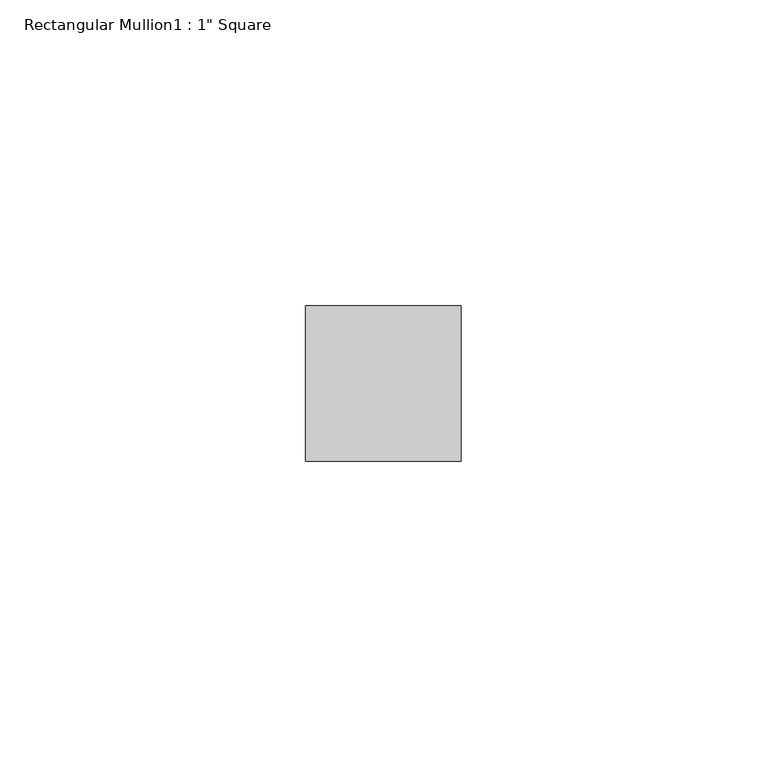
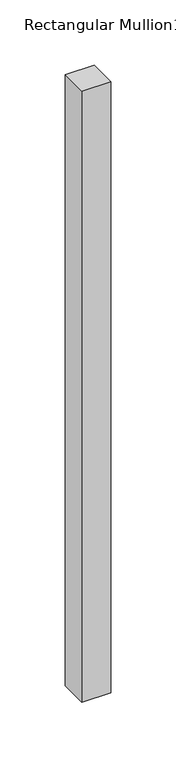
"""IFC4 building model written with IfcOpenShell, lengths in millimetres: member geometry."""

from ifc_helpers import new_model, si_unit, frame, origin, place, context, project, spatial, polyline, outline, extrude, source, transform, mapped, element, save


def member_8ca96f9c(model_context):
    return source(origin(), model_context, "Body", "SweptSolid", [
        extrude(outline(polyline([(12.7, -19.05), (12.7, -44.45), (-12.7, -44.45), (-12.7, -19.05), (12.7, -19.05)])), frame((0.0, 0.0, -571.5), z_axis=(0.0, 0.0, 1.0), x_axis=(1.0, 0.0, 0.0)), (0.0, 0.0, 1.0), 571.5),
    ])


if __name__ == "__main__":
    model = new_model("IFC4")
    model_context = context("Model", 3, world=origin())
    ifc_project = project(units=[si_unit("LENGTHUNIT", "METRE", prefix="MILLI")], contexts=[model_context])
    site = spatial("IfcSite", under=ifc_project)
    building = spatial("IfcBuilding", under=site)
    placement = place(None, origin())
    member_shape = member_8ca96f9c(model_context)
    element("IfcMember", 1, ObjectType="Rectangular Mullion1 : 1\" Square", at=placement, inside=building, context=model_context, shape_type="MappedRepresentation", body=[
        mapped(member_shape, transform((0.0, 0.0, 0.0), x_axis=(1.0, 0.0, 0.0), y_axis=(0.0, 1.0, 0.0), z_axis=(0.0, 0.0, 1.0))),
    ])
    save(model, "model.ifc")

# Revit data of these elements
# Type "Rectangular Mullion1 : 1\" Square"
#   built-in parameter 1007351 = 0.104167 (stored number, unit not read)
#   built-in parameter 1007304 = 0.0833333 (stored number, unit not read)
#   built-in parameter 1007301 = 0.0416667 (stored number, unit not read)
#   built-in parameter 1007300 = 0.0416667 (stored number, unit not read)
